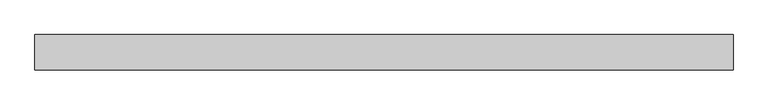
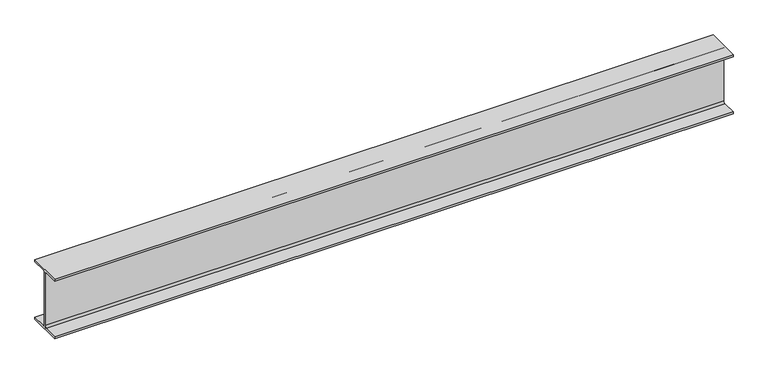
"""IFC4 building model written with IfcOpenShell, lengths in millimetres: beam geometry, Old_Steel Beam_H-KSD3502 : H_SB_ASB_H-200×200x8x12."""

from ifc_helpers import new_model, si_unit, point, frame, frame_2d, origin, place, context, project, spatial, polyline, circle_curve, trimmed, segment, composite_curve, outline, extrude, source, transform, mapped, element, save


def beam_5fd4a863(model_context):
    return source(origin(), model_context, "Body", "SweptSolid", [
        extrude(outline(composite_curve([segment(polyline([(82.5, -141.5), (82.5, -151.7), (-82.5, -151.7), (-82.5, -141.5), (-11.9, -141.5)]), True, "CONTINUOUS"), segment(trimmed(circle_curve(frame_2d((-11.9, -132.6)), 8.9), [point((-11.9, -141.5))], [point((-3.0, -132.6))], True, "CARTESIAN"), True, "CONTINUOUS"), segment(polyline([(-3.0, -132.6), (-3.0, 132.6)]), True, "CONTINUOUS"), segment(trimmed(circle_curve(frame_2d((-11.9, 132.6)), 8.9), [point((-3.0, 132.6))], [point((-11.9, 141.5))], True, "CARTESIAN"), True, "CONTINUOUS"), segment(polyline([(-11.9, 141.5), (-82.5, 141.5), (-82.5, 151.7), (82.5, 151.7), (82.5, 141.5), (11.9, 141.5)]), True, "CONTINUOUS"), segment(trimmed(circle_curve(frame_2d((11.9, 132.6)), 8.9), [point((11.9, 141.5))], [point((3.0, 132.6))], True, "CARTESIAN"), True, "CONTINUOUS"), segment(polyline([(3.0, 132.6), (3.0, -132.6)]), True, "CONTINUOUS"), segment(trimmed(circle_curve(frame_2d((11.9, -132.6)), 8.9), [point((3.0, -132.6))], [point((11.9, -141.5))], True, "CARTESIAN"), True, "CONTINUOUS"), segment(polyline([(11.9, -141.5), (82.5, -141.5)]), True, "CONTINUOUS")], self_intersect=False)), frame((-1689.2318964, 0.0, 0.0), z_axis=(1.0, 0.0, 0.0), x_axis=(0.0, 1.0, 0.0)), (0.0, 0.0, 1.0), 3273.7082384),
    ])


if __name__ == "__main__":
    model = new_model("IFC4")
    model_context = context("Model", 3, world=origin())
    ifc_project = project(units=[si_unit("LENGTHUNIT", "METRE", prefix="MILLI")], contexts=[model_context])
    site = spatial("IfcSite", under=ifc_project)
    building = spatial("IfcBuilding", under=site)
    placement = place(None, origin())
    beam_shape = beam_5fd4a863(model_context)
    element("IfcBeam", 1, ObjectType="Old_Steel Beam_H-KSD3502 : H_SB_ASB_H-200×200x8x12", at=placement, inside=building, context=model_context, shape_type="MappedRepresentation", body=[
        mapped(beam_shape, transform((0.0, 0.0, 0.0), x_axis=(1.0, 0.0, 0.0), y_axis=(0.0, 1.0, 0.0), z_axis=(0.0, 0.0, 1.0))),
    ])
    save(model, "model.ifc")

# Revit data of these elements
# Type "Old_Steel Beam_H-KSD3502 : H_SB_ASB_H-200×200x8x12"
#   Width = 20.0 cm
#   Web Thickness = 0.8 cm
#   Web Fillet = 1.3 cm
#   Warping Constant = 141376.0 cm⁶
#   Torsional Moment of Inertia = 26.2485 cm⁴
#   Torsional Modulus = 1.0 cm³
#   Section Area = 63.53 cm²
#   Plastic Modulus weak axis = 244.0 cm³
#   Plastic Modulus strong axis = 525.0 cm³
#   Perimeter = 1.16 m²/m
#   Nominal Weight = 49.90 kgf/m
#   Moment of Inertia weak axis = 1600.00 cm⁴
#   Moment of Inertia strong axis = 4720.00 cm⁴
#   Height = 20.0 cm
#   Flange Thickness = 1.2 cm
#   Elastic Modulus weak axis = 160.0 cm³
#   Elastic Modulus strong axis = 472.0 cm³
#   Centroid Vertical = 10.0 cm
#   Centroid Horizontal = 10.0 cm
#   Length [instance default] = 1.5240 m
#   Structural Material [instance default] = Steel, 45-345
#   Assembly Code = ""
# Element 1 (IfcBeam, "Old_Steel Beam_H-KSD3502 : H_SB_ASB_H-200×200x8x12")
#   Structural Material = none
# Materials
#   "Steel, 45-345": class "Metal", colour RGB 189 187 185, transparency 0, Description = "Steel 345 MPa", Cost = 0
